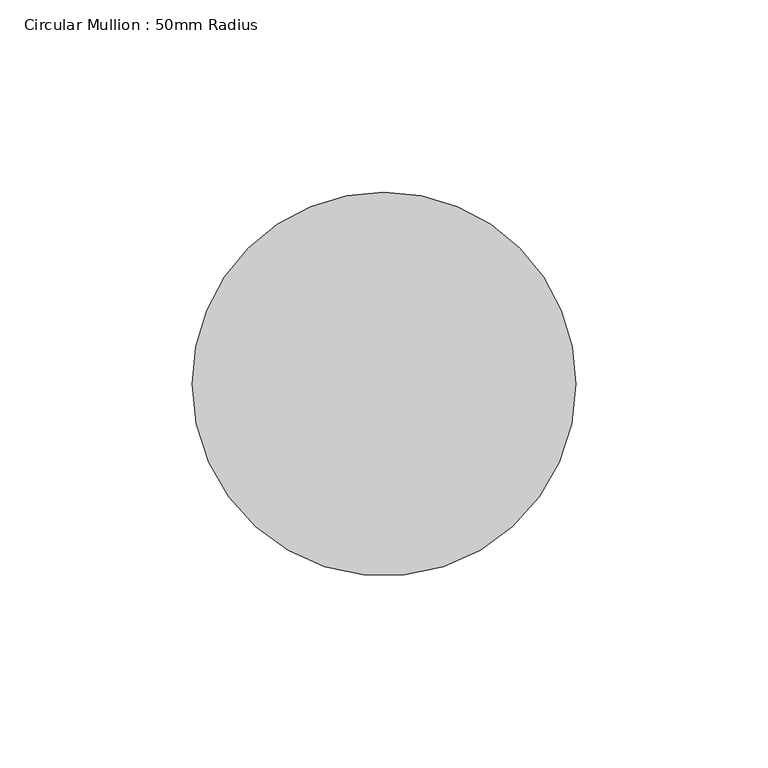
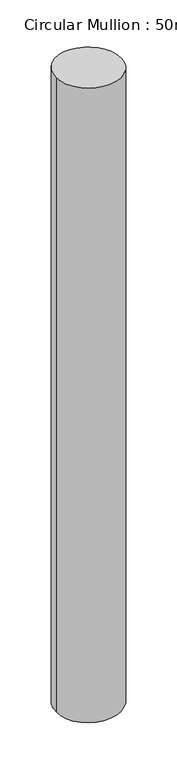
"""IFC4 building model written with IfcOpenShell, lengths in millimetres: member geometry, Circular Mullion : 50mm Radius."""

from ifc_helpers import new_model, si_unit, frame, origin, place, context, project, spatial, ellipse_curve, source, transform, mapped, element, save
from ifc_brep_helpers import plane_surface, cylinder_surface, advanced_brep


def circular_mullion_50mm_radius_98ae6d3a(model_context):
    return source(origin(), model_context, "Body", "AdvancedBrep", [
        advanced_brep(
        [(-100.0, 0.0, 2.1476675), (0.0, 0.0, 0.0), (0.0, 0.0, -1032.2495704), (-100.0, 0.0, -1034.3390242)],
        [
            (0, 1, ellipse_curve(frame((-50.0, 0.0, 1.0738337), z_axis=(-0.021466550257719808, -0.021949809729911254, -0.999528585420574), x_axis=(-0.6988631848040531, -0.71459613908724, 0.03070190429185324)), 50.0235818, 50.0)),
            (1, 2),
            (2, 3, ellipse_curve(frame((-50.0, 0.0, -1033.2942973), z_axis=(-0.020885214180050005, -0.021355386492789397, 0.9995537780912027), x_axis=(0.6988807993378675, 0.7146141501630517, 0.029870465406525937)), 50.0223211, 50.0)),
            (3, 0),
            (1, 0, ellipse_curve(frame((-50.0, 0.0, 1.0738337), z_axis=(-0.021466550257719808, -0.021949809729911254, -0.999528585420574), x_axis=(-0.6988631848040531, -0.71459613908724, 0.03070190429185324)), 50.0235818, 50.0)),
            (3, 2, ellipse_curve(frame((-50.0, 0.0, -1033.2942973), z_axis=(-0.020885214180050005, -0.021355386492789397, 0.9995537780912027), x_axis=(0.6988807993378675, 0.7146141501630517, 0.029870465406525937)), 50.0223211, 50.0)),
        ],
        [
            cylinder_surface(frame((-50.0, 0.0, 0.0), z_axis=(0.0, 0.0, 1.0), x_axis=(1.0, 0.0, 0.0)), 50.0),
            plane_surface(frame((-217.9116299, 213.1139638, 0.0), z_axis=(0.021466550257719808, 0.021949809729911254, 0.999528585420574), x_axis=(0.6988631848040535, 0.7145961390872393, -0.030701904291859764))),
            plane_surface(frame((-217.9116299, 213.1139638, -1032.2495704), z_axis=(0.020885214180050005, 0.021355386492789397, -0.9995537780912027), x_axis=(0.6988807993378674, 0.7146141501630517, 0.029870465406534485))),
        ],
        [
            (0, [[1, 2, 3, 4]]),
            (0, [[5, -4, 6, -2]]),
            (1, [[-1, -5]]),
            (2, [[-6, -3]]),
        ],
    ),
    ])


if __name__ == "__main__":
    model = new_model("IFC4")
    model_context = context("Model", 3, world=origin())
    ifc_project = project(units=[si_unit("LENGTHUNIT", "METRE", prefix="MILLI")], contexts=[model_context])
    site = spatial("IfcSite", under=ifc_project)
    building = spatial("IfcBuilding", under=site)
    placement = place(None, origin())
    circular_mullion_50mm_radius_shape = circular_mullion_50mm_radius_98ae6d3a(model_context)
    element("IfcMember", 1, ObjectType="Circular Mullion : 50mm Radius", at=placement, inside=building, context=model_context, shape_type="MappedRepresentation", body=[
        mapped(circular_mullion_50mm_radius_shape, transform((0.0, 0.0, 0.0), x_axis=(1.0, 0.0, 0.0), y_axis=(0.0, 1.0, 0.0), z_axis=(0.0, 0.0, 1.0))),
    ])
    save(model, "model.ifc")

# Revit data of these elements
# Type "Circular Mullion : 50mm Radius"
#   built-in parameter 1007350 = 0.164042 (stored number, unit not read)
# Element 1 (IfcMember, "Circular Mullion : 50mm Radius")
#   Materials on its faces: "Aluminium"
# Materials
#   "Aluminium": class "Metal", colour RGB 247 247 247, transparency 0, Description = "Aluminium 6061", Cost = 0
